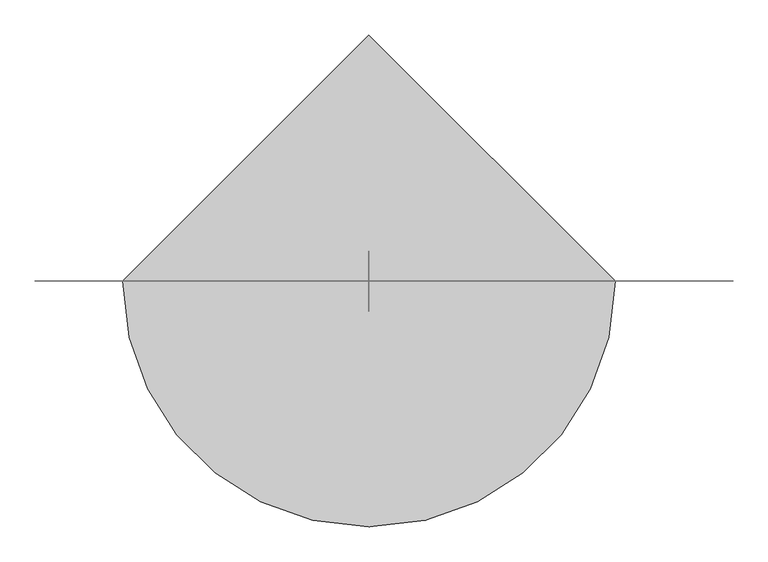
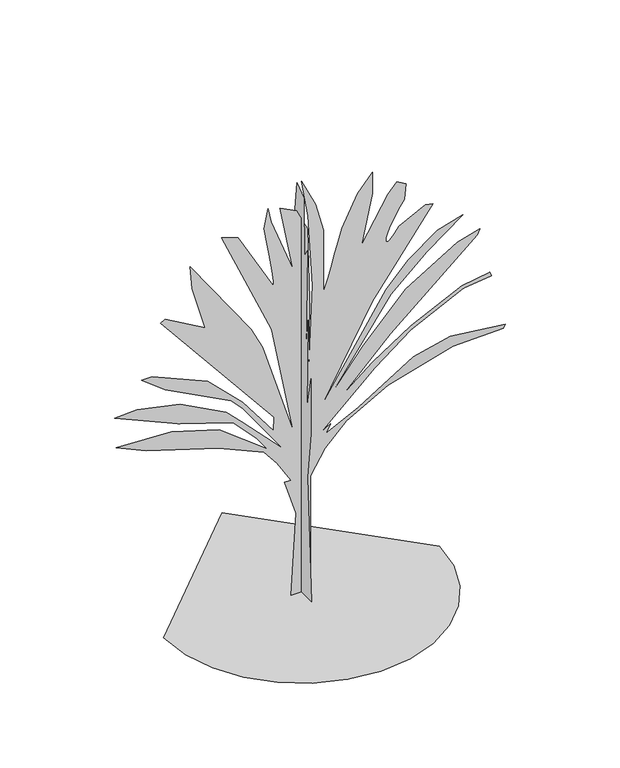
"""IFC4 building model written with IfcOpenShell, lengths in millimetres: proxy geometry, travelers palm 26121 : travelers palm 26121."""

from ifc_helpers import new_model, si_unit, origin, place, context, project, spatial, triangles, source, transform, mapped, element, save


def entourage_0177ab4a(model_context):
    return source(origin(), model_context, "Body", "Tessellation", [
        triangles([(-93.7534889, -0.0079219, 0.0614497), (-47.9158571, -0.0079683, 779.2394274), (-154.8704887, -0.0079884, 1115.3806829), (-93.7534889, -0.0079881, 1110.2879705), (-221.0799467, -0.0080005, 1319.1040764), (-343.3142189, -0.0080096, 1471.8953316), (-755.8511021, -0.0080203, 1650.1526196), (-1417.9506592, -0.0080327, 1858.9686527), (-1692.9744244, -0.0080403, 1986.2938751), (-1183.6685932, -0.0080388, 1960.827697), (-750.7583897, -0.0080309, 1828.4099075), (-312.7554374, -0.0080109, 1492.2660358), (-409.5244217, -0.008019, 1629.7791538), (-623.4331673, -0.0080324, 1853.8733242), (-1122.5511028, -0.0080421, 2016.8526203), (-1708.2550323, -0.0080576, 2276.5982483), (-1499.4389992, -0.0080582, 2286.7861439), (-1107.2729656, -0.008053, 2200.2026207), (-689.6408993, -0.0080397, 1976.1084503), (-547.0350326, -0.0080312, 1833.5026199), (-170.149607, -0.0080081, 1446.4291534), (-531.7569317, -0.0080385, 1955.7349846), (-643.8040169, -0.0080455, 2072.8773983), (-1244.7860836, -0.0080643, 2388.6453335), (-1458.6948292, -0.0080743, 2556.7145805), (-1361.9258812, -0.0080743, 2556.7145805), (-857.7127625, -0.0080609, 2332.6230263), (-536.8496078, -0.0080424, 2021.9453327), (-256.7306412, -0.00802, 1645.0599072), (-251.6384557, -0.0080279, 1777.4776966), (-1285.5302536, -0.0081034, 3045.6393883), (-1244.7860836, -0.008105, 3071.1157402), (-878.0860828, -0.0080922, 2857.1968208), (-1000.3185928, -0.0081174, 3279.9291573), (-1015.5992735, -0.0081302, 3493.8480766), (-460.4539802, -0.0080828, 2699.3102371), (-353.4996074, -0.00807, 2485.4142815), (-73.3816582, -0.0080157, 1573.756992), (-272.0112855, -0.0080789, 2633.1177658), (-730.3875401, -0.0081411, 3677.1854324), (-577.5937778, -0.0081377, 3621.1783859), (-261.8258789, -0.0081041, 3055.8248131), (-253.7766246, -0.0081039, 3053.36101), (-254.8154783, -0.0081061, 3089.6323425), (-263.4286335, -0.0081101, 3158.2124588), (-278.0996675, -0.0081158, 3252.5988487), (-297.3122485, -0.0081226, 3366.3907402), (-319.5550223, -0.0081301, 3493.0862045), (-343.3142189, -0.008138, 3626.2583084), (-302.5700489, -0.0081487, 3804.5157417), (-277.1039979, -0.0081408, 3672.1055099), (-78.4743615, -0.0081092, 3142.4134232), (-195.6149131, -0.0081469, 3773.9594673), (-42.8231537, -0.0081423, 3697.556282), (53.9453128, -0.0081299, 3488.742865), (74.3173933, -0.0080886, 2796.084272), (64.1312281, -0.008043, 2032.1306122), (99.7824359, -0.0080965, 2928.5200836), (59.0382705, -0.0081371, 3610.9929611), (3.0145246, -0.0081581, 3962.4023254), (130.3409359, -0.0081423, 3697.556282), (201.643851, -0.0081259, 3422.5503937), (201.643851, -0.008091, 2836.8259712), (206.54377, -0.0080912, 2840.5597549), (220.2640989, -0.0080935, 2878.5074387), (241.3341791, -0.0080974, 2944.9539642), (268.285114, -0.0081028, 3034.2095627), (299.6439739, -0.0081091, 3140.5594666), (333.9441513, -0.0081161, 3258.339196), (369.7149693, -0.0081235, 3381.7834053), (512.3208361, -0.0081405, 3667.0000076), (649.833954, -0.0081499, 3824.8865913), (649.833954, -0.0081377, 3621.1783859), (547.9722937, -0.0081101, 3157.7043503), (792.4397844, -0.0081341, 3560.0405479), (873.9281244, -0.0081399, 3656.8145828), (955.4164644, -0.0081368, 3605.8877495), (940.1383272, -0.0081283, 3463.2918022), (902.2287952, -0.0081247, 3401.3412231), (866.0592007, -0.008121, 3341.0669952), (833.3617779, -0.0081176, 3284.0693115), (805.8763916, -0.0081145, 3232.0248138), (785.3405085, -0.0081119, 3186.5842735), (773.4913771, -0.0081096, 3149.3731728), (772.066464, -0.008108, 3122.0428642), (778.9574678, -0.0081071, 3107.4885201), (790.3900549, -0.008107, 3106.0406433), (805.6096928, -0.0081076, 3115.4894852), (823.8595963, -0.0081087, 3133.6758751), (844.3802914, -0.0081102, 3158.4156441), (866.4147749, -0.0081119, 3187.5240417), (889.2062616, -0.0081138, 3218.8168991), (1133.6737524, -0.008121, 3341.0417061), (1199.8839552, -0.0081201, 3325.7763588), (649.833954, -0.0080755, 2577.0854301), (171.0856145, -0.0080239, 1711.2701099), (772.066464, -0.0080798, 2648.3834038), (975.7897848, -0.0080925, 2862.3023232), (1240.6281979, -0.0081041, 3055.8248131), (1474.9102638, -0.0081083, 3127.1480759), (1148.9544331, -0.0080937, 2882.6728821), (817.9058899, -0.0080761, 2587.2708549), (247.4814783, -0.0080279, 1777.4776966), (568.3456504, -0.0080521, 2184.9244835), (950.323752, -0.0080764, 2592.3763573), (1423.9781982, -0.0080934, 2877.5676704), (1632.7942314, -0.0080968, 2933.6000061), (1607.3281986, -0.008094, 2887.7783844), (812.810634, -0.0080537, 2210.3880455), (369.7149693, -0.0080272, 1767.2924171), (649.833954, -0.0080406, 1991.3865875), (1001.2558903, -0.0080543, 2220.5759411), (1464.7223682, -0.0080676, 2444.6699661), (1724.470467, -0.00807, 2485.4142815), (1734.6558918, -0.0080676, 2444.6699661), (1480.0029762, -0.0080658, 2414.1113663), (1001.2558903, -0.0080518, 2179.8317711), (670.2048037, -0.008037, 1930.2715679), (181.271766, -0.0080099, 1476.9878986), (267.853309, -0.0080133, 1533.012822), (227.1093933, -0.0080084, 1451.5218658), (522.5062245, -0.0080172, 1599.2204086), (1021.6266672, -0.0080361, 1914.9909599), (1362.8631786, -0.0080406, 1991.3865875), (1861.983585, -0.0080373, 1935.3642803), (1846.702977, -0.0080351, 1899.7128227), (1383.2340282, -0.0080345, 1889.5247818), (792.4397844, -0.0080242, 1716.3628223), (410.4591393, -0.0080118, 1507.5467892), (216.9232418, -0.0080002, 1314.0087479), (84.5035629, -0.0079872, 1095.0072899), (84.5035629, -0.0079219, 0.0), (0.0460873, 53.9902683, 0.0519176), (0.0460761, -156.8964007, 0.0519049), (0.0460873, -97.584823, 1166.5210207), (0.0460761, -150.306614, 1621.2474072), (0.0460761, -150.3063596, 2148.4652264), (0.0460873, -90.9945366, 1832.1335175), (0.0460873, -104.1746006, 2688.8710487), (0.0460873, -71.2236731, 2379.1228043), (0.0460873, -97.584823, 3354.4783859), (0.0460873, -51.4530639, 3275.3826324), (0.0460873, -44.8630274, 3828.9758766), (0.0460982, 67.1710998, 3908.0460503), (0.0460982, 133.0732182, 3374.239389), (0.0460982, 152.8438319, 2609.7752953), (0.0460982, 106.7123182, 1950.7591255), (0.0460873, 53.9902683, 1120.3895342), (-1259.0684967, 0.0, 0.0575648), (-1225.7818657, -288.495908, 0.0575478), (-1130.983873, -553.4307541, 0.0575321), (-982.2667877, -787.2201176, 0.0575181), (-787.2201176, -982.2667877, 0.0575064), (-553.4307541, -1130.983873, 0.0574975), (-288.495908, -1225.7818657, 0.0574919), (4.41e-05, -1259.0684967, 0.0574899), (288.495908, -1225.7818657, 0.0574919), (553.4307541, -1130.983873, 0.0574975), (787.2201176, -982.2667877, 0.0575064), (982.2667877, -787.2201176, 0.0575181), (1130.983873, -553.4307541, 0.0575321), (1225.7818657, -288.495908, 0.0575478), (1259.0684967, 0.0001101, 0.0575648), (-0.0001766, 1259.0684967, 0.05764)], [[59, 60, 61], [99, 100, 101], [8, 9, 10], [49, 50, 51], [98, 99, 101], [15, 16, 17], [15, 17, 18], [119, 120, 121], [34, 35, 36], [33, 34, 36], [98, 101, 102], [97, 98, 102], [24, 25, 26], [24, 26, 27], [23, 24, 27], [23, 27, 28], [22, 23, 28], [22, 28, 29], [21, 22, 29], [7, 8, 10], [7, 10, 11], [71, 72, 73], [106, 107, 108], [106, 108, 109], [105, 106, 109], [104, 105, 109], [104, 109, 110], [103, 104, 110], [39, 40, 41], [39, 41, 42], [52, 53, 54], [52, 54, 55], [52, 55, 56], [59, 61, 62], [58, 59, 62], [58, 62, 63], [57, 58, 63], [7, 11, 12], [6, 7, 12], [15, 18, 19], [14, 15, 19], [14, 19, 20], [13, 14, 20], [13, 20, 21], [12, 13, 21], [93, 94, 95], [92, 93, 95], [91, 92, 95], [90, 91, 95], [89, 90, 95], [88, 89, 95], [87, 88, 95], [2, 3, 4], [96, 97, 102], [96, 102, 103], [124, 125, 126], [124, 126, 127], [39, 42, 43], [49, 51, 52], [48, 49, 52], [47, 48, 52], [46, 47, 52], [45, 46, 52], [44, 45, 52], [86, 87, 95], [114, 115, 116], [113, 114, 116], [30, 31, 32], [30, 32, 33], [30, 33, 36], [30, 36, 37], [30, 37, 38], [29, 30, 38], [21, 29, 38], [131, 132, 1], [131, 1, 2], [131, 2, 4], [5, 6, 12], [5, 12, 21], [123, 124, 127], [123, 127, 128], [122, 123, 128], [122, 128, 129], [121, 122, 129], [121, 129, 130], [113, 116, 117], [112, 113, 117], [111, 112, 117], [111, 117, 118], [110, 111, 118], [110, 118, 119], [103, 110, 119], [96, 103, 119], [71, 73, 74], [70, 71, 74], [69, 70, 74], [68, 69, 74], [44, 52, 56], [43, 44, 56], [39, 43, 56], [39, 56, 57], [38, 39, 57], [75, 76, 77], [75, 77, 78], [74, 75, 78], [74, 78, 79], [74, 79, 80], [74, 80, 81], [74, 81, 82], [74, 82, 83], [74, 83, 84], [74, 84, 85], [67, 68, 74], [119, 121, 130], [130, 131, 4], [130, 4, 5], [130, 5, 21], [119, 130, 21], [119, 21, 38], [96, 119, 38], [96, 38, 57], [95, 96, 57], [95, 57, 63], [95, 63, 64], [86, 95, 64], [86, 64, 65], [86, 65, 66], [86, 66, 67], [86, 67, 74], [86, 74, 85], [138, 139, 140], [136, 137, 138], [140, 141, 142], [143, 144, 145], [142, 143, 145], [142, 145, 146], [140, 142, 146], [140, 146, 147], [138, 140, 147], [138, 147, 148], [136, 138, 148], [135, 136, 148], [134, 135, 148], [134, 148, 133], [163, 164, 149], [162, 163, 149], [162, 149, 150], [161, 162, 150], [161, 150, 151], [161, 151, 152], [160, 161, 152], [159, 160, 152], [159, 152, 153], [159, 153, 154], [159, 154, 155], [159, 155, 156], [159, 156, 157], [159, 157, 158]], closed=False),
    ])


if __name__ == "__main__":
    model = new_model("IFC4")
    model_context = context("Model", 3, world=origin())
    ifc_project = project(units=[si_unit("LENGTHUNIT", "METRE", prefix="MILLI")], contexts=[model_context])
    site = spatial("IfcSite", under=ifc_project)
    building = spatial("IfcBuilding", under=site)
    placement = place(None, origin())
    entourage_shape = entourage_0177ab4a(model_context)
    element("IfcBuildingElementProxy", 1, Name="travelers palm 26121 : travelers palm 26121", ObjectType="travelers palm 26121 : travelers palm 26121", at=placement, inside=building, context=model_context, shape_type="MappedRepresentation", body=[
        mapped(entourage_shape, transform((0.0, 0.0, 0.0), x_axis=(1.0, 0.0, 0.0), y_axis=(0.0, 1.0, 0.0), z_axis=(0.0, 0.0, 1.0))),
    ])
    save(model, "model.ifc")

# Revit data of these elements
# Project information
#   Project Issue Date = "Issue Date"
#   Project Status = "Project Status"
#   Client Name = "Owner"
#   Project Address = "640 West Main Street, Lake Geneva, WI 53147"
#   Project Name = "The Downtowner"
#   Project Number = "Project Number"
# Type "travelers palm 26121 : travelers palm 26121"
#   built-in parameter 1005195 = "RPC-16-G2M6-EAFX-C5H6-W000-ST1L-LVER-AU"
#   Height = 0
